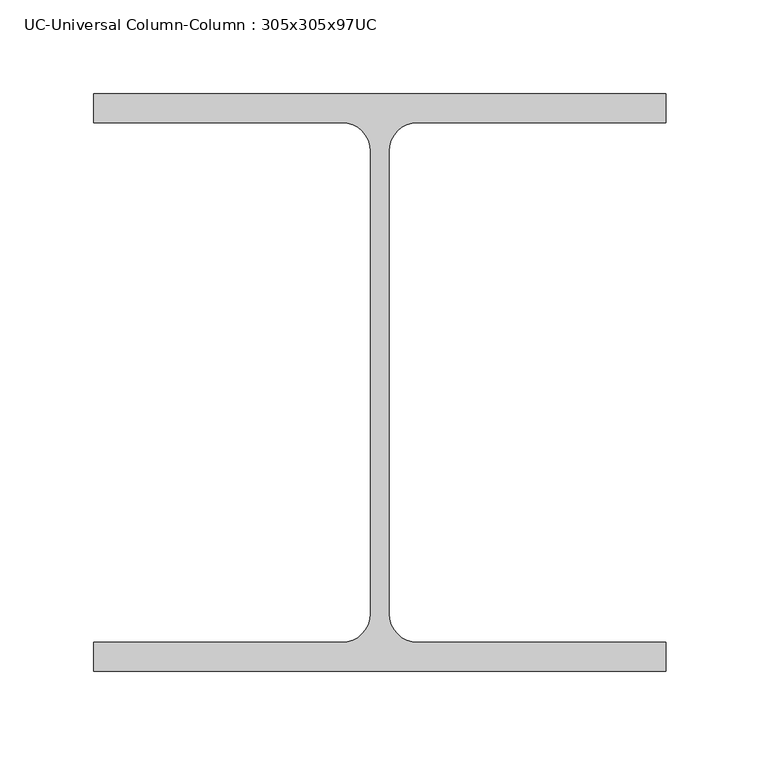
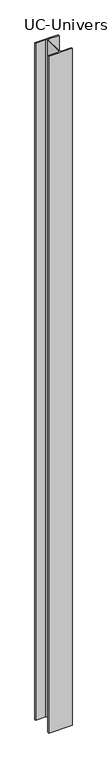
"""IFC4 building model written with IfcOpenShell, lengths in millimetres: column geometry, UC-Universal Column-Column : 305x305x97UC."""

from ifc_helpers import new_model, si_unit, point, frame, frame_2d, origin, place, context, project, spatial, polyline, circle_curve, trimmed, segment, composite_curve, outline, extrude, source, transform, mapped, element, save


def uc_universal_column_column_305x305x97uc_8da79b43(model_context):
    return source(origin(), model_context, "Body", "SweptSolid", [
        extrude(outline(composite_curve([segment(polyline([(152.65, -153.95), (-152.65, -153.95), (-152.65, -138.55), (-20.15, -138.55)]), True, "CONTINUOUS"), segment(trimmed(circle_curve(frame_2d((-20.15, -123.35)), 15.2), [point((-20.15, -138.55))], [point((-4.95, -123.35))], True, "CARTESIAN"), True, "CONTINUOUS"), segment(polyline([(-4.95, -123.35), (-4.95, 123.35)]), True, "CONTINUOUS"), segment(trimmed(circle_curve(frame_2d((-20.15, 123.35)), 15.2), [point((-4.95, 123.35))], [point((-20.15, 138.55))], True, "CARTESIAN"), True, "CONTINUOUS"), segment(polyline([(-20.15, 138.55), (-152.65, 138.55), (-152.65, 153.95), (152.65, 153.95), (152.65, 138.55), (20.15, 138.55)]), True, "CONTINUOUS"), segment(trimmed(circle_curve(frame_2d((20.15, 123.35)), 15.2), [point((20.15, 138.55))], [point((4.95, 123.35))], True, "CARTESIAN"), True, "CONTINUOUS"), segment(polyline([(4.95, 123.35), (4.95, -123.35)]), True, "CONTINUOUS"), segment(trimmed(circle_curve(frame_2d((20.15, -123.35)), 15.2), [point((4.95, -123.35))], [point((20.15, -138.55))], True, "CARTESIAN"), True, "CONTINUOUS"), segment(polyline([(20.15, -138.55), (152.65, -138.55), (152.65, -153.95)]), True, "CONTINUOUS")], self_intersect=False)), frame((0.0, 0.0, -1500.0), z_axis=(0.0, 0.0, 1.0), x_axis=(1.0, 0.0, 0.0)), (0.0, 0.0, 1.0), 9300.0),
    ])


if __name__ == "__main__":
    model = new_model("IFC4")
    model_context = context("Model", 3, world=origin())
    ifc_project = project(units=[si_unit("LENGTHUNIT", "METRE", prefix="MILLI")], contexts=[model_context])
    site = spatial("IfcSite", under=ifc_project)
    building = spatial("IfcBuilding", under=site)
    placement = place(None, origin())
    uc_universal_column_column_305x305x97uc_shape = uc_universal_column_column_305x305x97uc_8da79b43(model_context)
    element("IfcColumn", 1, ObjectType="UC-Universal Column-Column : 305x305x97UC", at=placement, inside=building, context=model_context, shape_type="MappedRepresentation", body=[
        mapped(uc_universal_column_column_305x305x97uc_shape, transform((0.0, 0.0, 0.0), x_axis=(1.0, 0.0, 0.0), y_axis=(0.0, 1.0, 0.0), z_axis=(0.0, 0.0, 1.0))),
    ])
    save(model, "model.ifc")

# Revit data of these elements
# Type "UC-Universal Column-Column : 305x305x97UC"
#   Keynote = "G10"
#   Nominal h = ""
#   W = 0
#   Ix = 0
#   M = 96.9
#   Zx = 0
#   b = 305.3 mm
#   h = 307.9 mm
#   r = 15.2 mm
#   s = 9.9 mm
#   t = 15.4 mm
#   A = 123 m²
#   Structural Material [instance default] = Steel, 45-345
#   Assembly Code = ""
# Element 1 (IfcColumn, "UC-Universal Column-Column : 305x305x97UC")
#   Materials on its faces: "Steel, 45-345"
# Materials
#   "Steel, 45-345": class "Metal", colour RGB 247 247 247, transparency 0, Description = "Steel 345 MPa", Cost = 0
